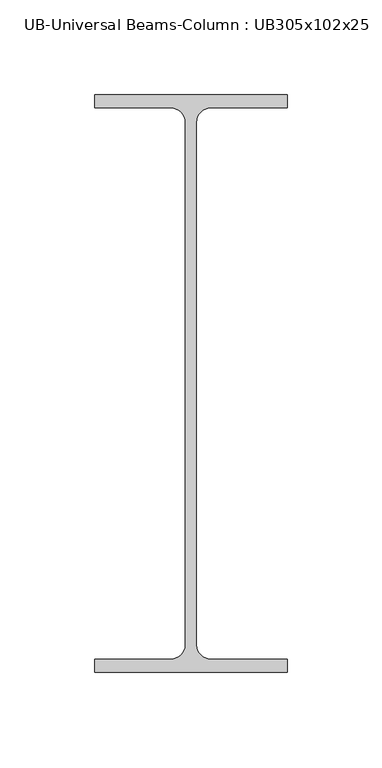
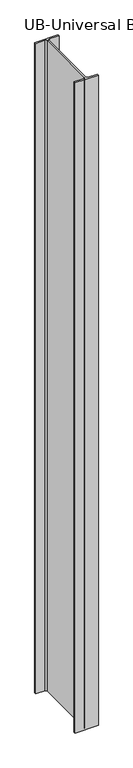
"""IFC4 building model written with IfcOpenShell, lengths in millimetres: column geometry, UB-Universal Beams-Column : UB305x102x25."""

from ifc_helpers import new_model, si_unit, point, frame_2d, origin, origin_with_axes, place, context, project, spatial, polyline, circle_curve, trimmed, segment, composite_curve, outline, extrude, source, transform, mapped, element, save


def ub_universal_beams_column_ub305x102x25_abf45cfe(model_context):
    return source(origin(), model_context, "Body", "SweptSolid", [
        extrude(outline(composite_curve([segment(polyline([(50.8, 152.55), (50.8, 145.55), (10.5, 145.55)]), True, "CONTINUOUS"), segment(trimmed(circle_curve(frame_2d((10.5, 137.95)), 7.6), [point((10.5, 145.55))], [point((2.9, 137.95))], True, "CARTESIAN"), True, "CONTINUOUS"), segment(polyline([(2.9, 137.95), (2.9, -137.95)]), True, "CONTINUOUS"), segment(trimmed(circle_curve(frame_2d((10.5, -137.95)), 7.6), [point((2.9, -137.95))], [point((10.5, -145.55))], True, "CARTESIAN"), True, "CONTINUOUS"), segment(polyline([(10.5, -145.55), (50.8, -145.55), (50.8, -152.55), (-50.8, -152.55), (-50.8, -145.55), (-10.5, -145.55)]), True, "CONTINUOUS"), segment(trimmed(circle_curve(frame_2d((-10.5, -137.95)), 7.6), [point((-10.5, -145.55))], [point((-2.9, -137.95))], True, "CARTESIAN"), True, "CONTINUOUS"), segment(polyline([(-2.9, -137.95), (-2.9, 137.95)]), True, "CONTINUOUS"), segment(trimmed(circle_curve(frame_2d((-10.5, 137.95)), 7.6), [point((-2.9, 137.95))], [point((-10.5, 145.55))], True, "CARTESIAN"), True, "CONTINUOUS"), segment(polyline([(-10.5, 145.55), (-50.8, 145.55), (-50.8, 152.55), (50.8, 152.55)]), True, "CONTINUOUS")], self_intersect=False)), origin_with_axes(), (0.0, 0.0, 1.0), 3000.0),
    ])


if __name__ == "__main__":
    model = new_model("IFC4")
    model_context = context("Model", 3, world=origin())
    ifc_project = project(units=[si_unit("LENGTHUNIT", "METRE", prefix="MILLI")], contexts=[model_context])
    site = spatial("IfcSite", under=ifc_project)
    building = spatial("IfcBuilding", under=site)
    placement = place(None, origin())
    ub_universal_beams_column_ub305x102x25_shape = ub_universal_beams_column_ub305x102x25_abf45cfe(model_context)
    element("IfcColumn", 1, ObjectType="UB-Universal Beams-Column : UB305x102x25", at=placement, inside=building, context=model_context, shape_type="MappedRepresentation", body=[
        mapped(ub_universal_beams_column_ub305x102x25_shape, transform((0.0, 0.0, 0.0), x_axis=(1.0, 0.0, 0.0), y_axis=(0.0, 1.0, 0.0), z_axis=(0.0, 0.0, 1.0))),
    ])
    save(model, "model.ifc")

# Revit data of these elements
# Type "UB-Universal Beams-Column : UB305x102x25"
#   Section Name Key = "UB305X102X25"
#   Width = 101.6 mm
#   Web Thickness = 5.8 mm
#   Web Fillet = 7.6 mm
#   Warping Constant = 27300 cm⁶
#   Torsional Moment of Inertia = 4.77 cm⁴
#   Section Area = 31.6 cm²
#   Plastic Modulus weak axis = 0.00137727 (stored number, unit not read)
#   Plastic Modulus strong axis = 0.0120776 (stored number, unit not read)
#   Nominal Weight = 243.204 N/m
#   Moment of Inertia weak axis = 123 cm⁴
#   Moment of Inertia strong axis = 4455 cm⁴
#   Height = 305.1 mm
#   Flange Thickness = 7 mm
#   Elastic Modulus weak axis = 0.000854615 (stored number, unit not read)
#   Elastic Modulus strong axis = 0.0103119 (stored number, unit not read)
#   Centroid Vertical = 152.55 mm
#   Centroid Horizontal = 50.8 mm
#   Structural Material [instance default] = Metal - Steel 43-275
#   Type Comments = ""
#   Assembly Code = ""
# Element 1 (IfcColumn, "UB-Universal Beams-Column : UB305x102x25")
#   Materials on its faces: "Metal - Steel 43-275"
# Materials
#   "Metal - Steel 43-275": class "Metal", colour RGB 247 247 247, transparency 0, Cost = 0
